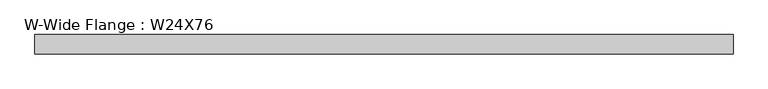
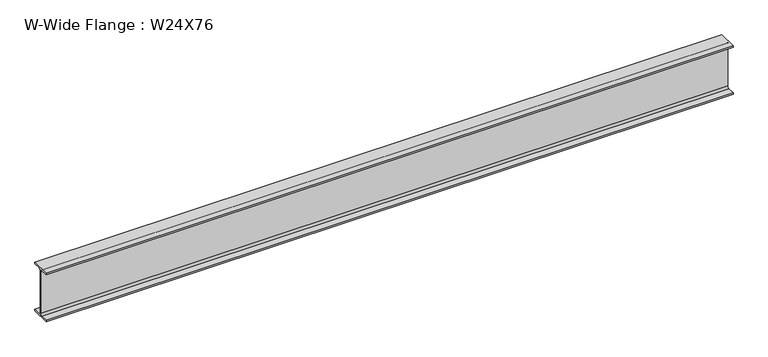
"""IFC4 building model written with IfcOpenShell, lengths in millimetres: beam geometry, W-Wide Flange : W24X76."""

from ifc_helpers import new_model, si_unit, point, frame, frame_2d, origin, place, context, project, spatial, polyline, circle_curve, trimmed, segment, composite_curve, outline, extrude, source, transform, mapped, element, save


def w_wide_flange_w24x76_8d3d20ef(model_context):
    return source(origin(), model_context, "Body", "SweptSolid", [
        extrude(outline(composite_curve([segment(polyline([(114.173, -286.258), (114.173, -303.53), (-114.173, -303.53), (-114.173, -286.258), (-28.0035, -286.258)]), True, "CONTINUOUS"), segment(trimmed(circle_curve(frame_2d((-28.0035, -263.8425)), 22.4155), [point((-28.0035, -286.258))], [point((-5.588, -263.8425))], True, "CARTESIAN"), True, "CONTINUOUS"), segment(polyline([(-5.588, -263.8425), (-5.588, 263.8425)]), True, "CONTINUOUS"), segment(trimmed(circle_curve(frame_2d((-28.0035, 263.8425)), 22.4155), [point((-5.588, 263.8425))], [point((-28.0035, 286.258))], True, "CARTESIAN"), True, "CONTINUOUS"), segment(polyline([(-28.0035, 286.258), (-114.173, 286.258), (-114.173, 303.53), (114.173, 303.53), (114.173, 286.258), (28.0035, 286.258)]), True, "CONTINUOUS"), segment(trimmed(circle_curve(frame_2d((28.0035, 263.8425)), 22.4155), [point((28.0035, 286.258))], [point((5.588, 263.8425))], True, "CARTESIAN"), True, "CONTINUOUS"), segment(polyline([(5.588, 263.8425), (5.588, -263.8425)]), True, "CONTINUOUS"), segment(trimmed(circle_curve(frame_2d((28.0035, -263.8425)), 22.4155), [point((5.588, -263.8425))], [point((28.0035, -286.258))], True, "CARTESIAN"), True, "CONTINUOUS"), segment(polyline([(28.0035, -286.258), (114.173, -286.258)]), True, "CONTINUOUS")], self_intersect=False)), frame((-4076.7, 0.0, 0.0), z_axis=(1.0, 0.0, 0.0), x_axis=(0.0, 1.0, 0.0)), (0.0, 0.0, 1.0), 8153.4),
    ])


if __name__ == "__main__":
    model = new_model("IFC4")
    model_context = context("Model", 3, world=origin())
    ifc_project = project(units=[si_unit("LENGTHUNIT", "METRE", prefix="MILLI")], contexts=[model_context])
    site = spatial("IfcSite", under=ifc_project)
    building = spatial("IfcBuilding", under=site)
    placement = place(None, origin())
    w_wide_flange_w24x76_shape = w_wide_flange_w24x76_8d3d20ef(model_context)
    element("IfcBeam", 1, ObjectType="W-Wide Flange : W24X76", at=placement, inside=building, context=model_context, shape_type="MappedRepresentation", body=[
        mapped(w_wide_flange_w24x76_shape, transform((0.0, 0.0, 0.0), x_axis=(1.0, 0.0, 0.0), y_axis=(0.0, 1.0, 0.0), z_axis=(0.0, 0.0, 1.0))),
    ])
    save(model, "model.ifc")

# Revit data of these elements
# Type "W-Wide Flange : W24X76"
#   Assembly Code = "B10"
#   W = 76
#   Length [instance default] = 5' - 0"
#   bf = 0' - 8.99"
#   d = 1' - 11.9"
#   k = 0' - 1 9/16"
#   k2 = 0' - 0.8825"
#   tf = 0' - 0.68"
#   tw = 0' - 0.44"
#   A = 0.155556 SF
#   Structural Material [instance default] = Steel ASTM A992
# Element 1 (IfcBeam, "W-Wide Flange : W24X76")
#   Materials on its faces: "Steel ASTM A992"
# Materials
#   "Steel ASTM A992": class "Metal", colour RGB 199 199 199, transparency 0, Description = "Structural steel 50ksi", Cost = 0
